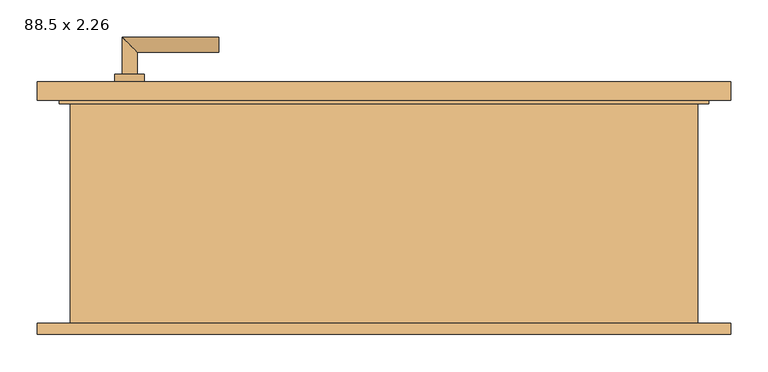
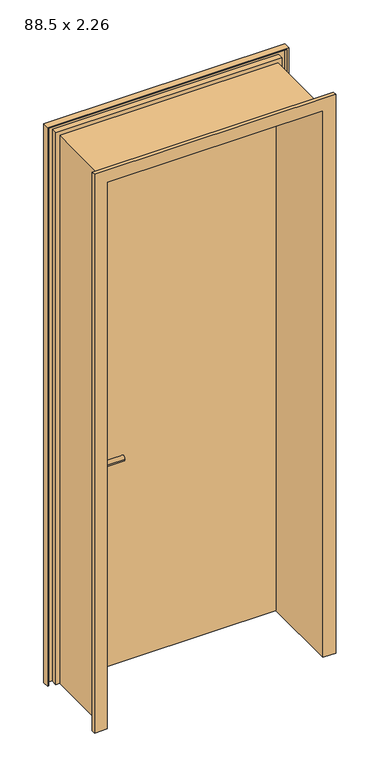
"""IFC4 building model written with IfcOpenShell, lengths in millimetres: door geometry, Drehflügel 1-flg - Stahlzarge : 88.5 x 2.26."""

from ifc_helpers import new_model, si_unit, point, frame, frame_2d, origin, place, context, project, spatial, polyline, circle_curve, ellipse_curve, trimmed, segment, composite_curve, outline, extrude, faceted_brep, source, transform, mapped, element, save
from ifc_brep_helpers import plane_surface, cylinder_surface, advanced_brep


def door_88_5_x_2_26_ba7bfb9e(model_context):
    return source(origin(), model_context, "Body", "SolidModel", [
        advanced_brep(
        [(-352.5, 139.4346141, 1000.0), (-332.5, 139.4346141, 1000.0), (-352.5, 69.4346141, 1000.0), (-332.5, 89.4346141, 1000.0), (-222.5, 69.4346141, 1000.0), (-222.5, 89.4346141, 1000.0)],
        [
            (0, 1, circle_curve(frame((-342.5, 139.4346141, 1000.0), z_axis=(0.0, 1.0, 0.0), x_axis=(1.0, 0.0, 0.0)), 10.0)),
            (1, 0, circle_curve(frame((-342.5, 139.4346141, 1000.0), z_axis=(0.0, 1.0, 0.0), x_axis=(1.0, 0.0, 0.0)), 10.0)),
            (0, 2),
            (2, 3, ellipse_curve(frame((-342.5, 79.4346141, 1000.0), z_axis=(-0.7071067811865385, 0.7071067811865565, 0.0), x_axis=(0.7071067811865563, 0.7071067811865386, 0.0)), 14.1421356, 10.0)),
            (3, 1),
            (3, 2, ellipse_curve(frame((-342.5, 79.4346141, 1000.0), z_axis=(-0.7071067811865385, 0.7071067811865565, 0.0), x_axis=(0.7071067811865563, 0.7071067811865386, 0.0)), 14.1421356, 10.0)),
            (4, 5, circle_curve(frame((-222.5, 79.4346141, 1000.0), z_axis=(1.0, 0.0, 0.0), x_axis=(0.0, 1.0, 0.0)), 10.0)),
            (5, 4, circle_curve(frame((-222.5, 79.4346141, 1000.0), z_axis=(1.0, 0.0, 0.0), x_axis=(0.0, 1.0, 0.0)), 10.0)),
            (2, 4),
            (5, 3),
        ],
        [
            plane_surface(frame((-342.5, 139.4346141, -287.7526403), z_axis=(0.0, 1.0, 0.0), x_axis=(0.0, 0.0, 1.0))),
            cylinder_surface(frame((-342.5, 139.4346141, 1000.0), z_axis=(0.0, 1.0, 0.0), x_axis=(1.0, 0.0, 0.0)), 10.0),
            plane_surface(frame((-222.5, 79.4346141, -287.7526403), z_axis=(1.0, 0.0, 0.0), x_axis=(0.0, 0.0, 1.0))),
            cylinder_surface(frame((-342.5, 79.4346141, 1000.0), z_axis=(-1.0, 0.0, 0.0), x_axis=(0.0, 1.0, 0.0)), 10.0),
        ],
        [
            (0, [[1, 2]]),
            (1, [[-1, 3, 4, 5]]),
            (1, [[-2, -5, 6, -3]]),
            (2, [[7, 8]]),
            (3, [[-4, 9, -8, 10]]),
            (3, [[-6, -10, -7, -9]]),
        ],
    ),
        advanced_brep(
        [(-332.5, 199.4346141, 1000.0), (-352.5, 199.4346141, 1000.0), (-332.5, 229.4346141, 1000.0), (-352.5, 249.4346141, 1000.0), (-222.5, 229.4346141, 1000.0), (-222.5, 249.4346141, 1000.0)],
        [
            (0, 1, circle_curve(frame((-342.5, 199.4346141, 1000.0), z_axis=(0.0, -1.0, 0.0), x_axis=(-1.0, 0.0, 0.0)), 10.0)),
            (1, 0, circle_curve(frame((-342.5, 199.4346141, 1000.0), z_axis=(0.0, -1.0, 0.0), x_axis=(-1.0, 0.0, 0.0)), 10.0)),
            (0, 2),
            (2, 3, ellipse_curve(frame((-342.5, 239.4346141, 1000.0), z_axis=(-0.7071067811865475, -0.7071067811865475, 0.0), x_axis=(0.7071067811865474, -0.7071067811865476, 0.0)), 14.1421356, 10.0)),
            (3, 1),
            (3, 2, ellipse_curve(frame((-342.5, 239.4346141, 1000.0), z_axis=(-0.7071067811865475, -0.7071067811865475, 0.0), x_axis=(0.7071067811865474, -0.7071067811865476, 0.0)), 14.1421356, 10.0)),
            (4, 5, circle_curve(frame((-222.5, 239.4346141, 1000.0), z_axis=(1.0, 0.0, 0.0), x_axis=(0.0, 1.0, 0.0)), 10.0)),
            (5, 4, circle_curve(frame((-222.5, 239.4346141, 1000.0), z_axis=(1.0, 0.0, 0.0), x_axis=(0.0, 1.0, 0.0)), 10.0)),
            (2, 4),
            (5, 3),
        ],
        [
            plane_surface(frame((-342.5, 199.4346141, -287.7526403), z_axis=(0.0, -1.0, 0.0), x_axis=(0.0, 0.0, 1.0))),
            cylinder_surface(frame((-342.5, 199.4346141, 1000.0), z_axis=(0.0, -1.0, 0.0), x_axis=(-1.0, 0.0, 0.0)), 10.0),
            plane_surface(frame((-222.5, 239.4346141, -287.7526403), z_axis=(1.0, 0.0, 0.0), x_axis=(0.0, 0.0, 1.0))),
            cylinder_surface(frame((-342.5, 239.4346141, 1000.0), z_axis=(-1.0, 0.0, 0.0), x_axis=(0.0, 1.0, 0.0)), 10.0),
        ],
        [
            (0, [[1, 2]]),
            (1, [[-1, 3, 4, 5]]),
            (1, [[-2, -5, 6, -3]]),
            (2, [[7, 8]]),
            (3, [[-4, 9, -8, 10]]),
            (3, [[-6, -10, -7, -9]]),
        ],
    ),
        extrude(outline(composite_curve([segment(trimmed(circle_curve(frame_2d((1000.0, -342.5)), 20.0), [point((1000.0, -362.5))], [point((1000.0, -322.5))], False, "CARTESIAN"), True, "CONTINUOUS"), segment(trimmed(circle_curve(frame_2d((1000.0, -342.5)), 20.0), [point((1000.0, -322.5))], [point((1000.0, -362.5))], False, "CARTESIAN"), True, "CONTINUOUS")], self_intersect=False)), frame((0.0, 129.4346141, 0.0), z_axis=(0.0, 1.0, 0.0), x_axis=(0.0, 0.0, 1.0)), (0.0, 0.0, 1.0), 10.0),
        extrude(outline(composite_curve([segment(trimmed(circle_curve(frame_2d((1000.0, -342.5)), 20.0), [point((1000.0, -362.5))], [point((1000.0, -322.5))], False, "CARTESIAN"), True, "CONTINUOUS"), segment(trimmed(circle_curve(frame_2d((1000.0, -342.5)), 20.0), [point((1000.0, -322.5))], [point((1000.0, -362.5))], False, "CARTESIAN"), True, "CONTINUOUS")], self_intersect=False)), frame((0.0, 189.4346141, 0.0), z_axis=(0.0, 1.0, 0.0), x_axis=(0.0, 0.0, 1.0)), (0.0, 0.0, 1.0), 10.0),
        extrude(outline(polyline([(432.5, 164.4346141), (-432.5, 164.4346141), (-432.5, 189.4346141), (432.5, 189.4346141), (432.5, 164.4346141)])), frame((0.0, 0.0, 100.0), z_axis=(0.0, 0.0, 1.0), x_axis=(1.0, 0.0, 0.0)), (0.0, 0.0, 1.0), 2250.0),
        faceted_brep([(466.9603207, -150.5653859, 100.0), (417.5, -150.5653859, 100.0), (417.5, 164.4346141, 100.0), (432.5, 164.4346141, 100.0), (432.5, 189.4346141, 100.0), (466.9603207, 189.4346141, 100.0), (466.9603207, 164.4346141, 100.0), (461.9603207, 164.4346141, 100.0), (461.9603207, 184.4346141, 100.0), (437.5, 184.4346141, 100.0), (437.5, 159.4346141, 100.0), (422.5, 159.4346141, 100.0), (422.5, -145.5653859, 100.0), (461.9603207, -145.5653859, 100.0), (461.9603207, -135.5653859, 100.0), (466.9603207, -135.5653859, 100.0), (466.9603207, -150.5653859, 2384.4603207), (-466.9603207, -150.5653859, 2384.4603207), (-466.9603207, -150.5653859, 100.0), (-417.5, -150.5653859, 100.0), (-417.5, -150.5653859, 2335.0), (417.5, -150.5653859, 2335.0), (417.5, 164.4346141, 2335.0), (-417.5, 164.4346141, 2335.0), (-417.5, 164.4346141, 100.0), (-432.5, 164.4346141, 100.0), (-432.5, 164.4346141, 2350.0), (432.5, 164.4346141, 2350.0), (432.5, 189.4346141, 2350.0), (-432.5, 189.4346141, 2350.0), (-432.5, 189.4346141, 100.0), (-466.9603207, 189.4346141, 100.0), (-466.9603207, 189.4346141, 2384.4603207), (466.9603207, 189.4346141, 2384.4603207), (466.9603207, 164.4346141, 2384.4603207), (-466.9603207, 164.4346141, 2384.4603207), (-466.9603207, 164.4346141, 100.0), (-461.9603207, 164.4346141, 100.0), (-461.9603207, 164.4346141, 2379.4603207), (461.9603207, 164.4346141, 2379.4603207), (461.9603207, 184.4346141, 2379.4603207), (-461.9603207, 184.4346141, 2379.4603207), (-461.9603207, 184.4346141, 100.0), (-437.5, 184.4346141, 100.0), (-437.5, 184.4346141, 2355.0), (437.5, 184.4346141, 2355.0), (437.5, 159.4346141, 2355.0), (-437.5, 159.4346141, 2355.0), (-437.5, 159.4346141, 100.0), (-422.5, 159.4346141, 100.0), (-422.5, 159.4346141, 2340.0), (422.5, 159.4346141, 2340.0), (422.5, -145.5653859, 2340.0), (-422.5, -145.5653859, 2340.0), (-422.5, -145.5653859, 100.0), (-461.9603207, -145.5653859, 100.0), (-461.9603207, -145.5653859, 2379.4603207), (461.9603207, -145.5653859, 2379.4603207), (461.9603207, -135.5653859, 2379.4603207), (-461.9603207, -135.5653859, 2379.4603207), (-461.9603207, -135.5653859, 100.0), (-466.9603207, -135.5653859, 100.0), (-466.9603207, -135.5653859, 2384.4603207), (466.9603207, -135.5653859, 2384.4603207)], [[[0, 1, 2, 3, 4, 5, 6, 7, 8, 9, 10, 11, 12, 13, 14, 15]], [[1, 0, 16, 17, 18, 19, 20, 21]], [[2, 1, 21, 22]], [[3, 2, 22, 23, 24, 25, 26, 27]], [[4, 3, 27, 28]], [[5, 4, 28, 29, 30, 31, 32, 33]], [[6, 5, 33, 34]], [[7, 6, 34, 35, 36, 37, 38, 39]], [[8, 7, 39, 40]], [[9, 8, 40, 41, 42, 43, 44, 45]], [[10, 9, 45, 46]], [[11, 10, 46, 47, 48, 49, 50, 51]], [[12, 11, 51, 52]], [[13, 12, 52, 53, 54, 55, 56, 57]], [[14, 13, 57, 58]], [[15, 14, 58, 59, 60, 61, 62, 63]], [[0, 15, 63, 16]], [[17, 62, 61, 18]], [[18, 61, 60, 55, 54, 49, 48, 43, 42, 37, 36, 31, 30, 25, 24, 19]], [[23, 20, 19, 24]], [[29, 26, 25, 30]], [[35, 32, 31, 36]], [[41, 38, 37, 42]], [[47, 44, 43, 48]], [[53, 50, 49, 54]], [[59, 56, 55, 60]], [[22, 21, 20, 23]], [[28, 27, 26, 29]], [[34, 33, 32, 35]], [[40, 39, 38, 41]], [[46, 45, 44, 47]], [[52, 51, 50, 53]], [[58, 57, 56, 59]], [[16, 63, 62, 17]]]),
    ])


if __name__ == "__main__":
    model = new_model("IFC4")
    model_context = context("Model", 3, world=origin())
    ifc_project = project(units=[si_unit("LENGTHUNIT", "METRE", prefix="MILLI")], contexts=[model_context])
    site = spatial("IfcSite", under=ifc_project)
    building = spatial("IfcBuilding", under=site)
    placement = place(None, origin())
    door_88_5_x_2_26_shape = door_88_5_x_2_26_ba7bfb9e(model_context)
    element("IfcDoor", 1, ObjectType="Drehflügel 1-flg - Stahlzarge : 88.5 x 2.26", at=placement, inside=building, context=model_context, shape_type="MappedRepresentation", body=[
        mapped(door_88_5_x_2_26_shape, transform((0.0, 0.0, 0.0), x_axis=(1.0, 0.0, 0.0), y_axis=(0.0, 1.0, 0.0), z_axis=(0.0, 0.0, 1.0))),
    ])
    save(model, "model.ifc")

# Revit data of these elements
# Type "Drehflügel 1-flg - Stahlzarge : 88.5 x 2.26"
#   Construction Type Id = "MDOOR"
#   Type Mark = "20"
#   Operation = "SingleSwingRight"
#   Keynote = "16.03"
#   Analytic Construction = "Metall"
#   Thermal Resistance (R) = 0.270117 (m²·K)/W
#   Heat Transfer Coefficient (U) = 3.7021 W/(m²·K)
#   Rough Width = 0.885 m
#   Rough Height [instance default] = 2.360 m
#   Höhe Türgriff [instance default] = 0.900 m
#   Height = 2.260 m
#   Fußbodenaufbau [instance default] = 0.100 m
#   Width = 0.885 m
#   Sichtbarkeit Sturzlinien [instance default] = yes
#   Türgriff auswählen [instance default] = element 221079
#   Türgriff [instance default] = none
#   Türflügel [instance default] = none
#   Rahmen/Pfosten [instance default] = Metall - Lackiert - Grau
#   Visual Light Transmittance = 0
#   Solar Heat Gain Coefficient = 0
#   Function = (empty or 0)
#   Wall Closure = (empty or 0)
# Element 1 (IfcDoor, "Drehflügel 1-flg - Stahlzarge : 88.5 x 2.26")
#   Materials on its faces: "Metall - Lackiert - Grau", "Metall - Chrom", "Holz - Birke"
# Materials
#   "Metall - Lackiert - Grau": class "Farbe 1", colour RGB 98 98 98, transparency 0, Cost = 0
#   "Metall - Chrom": class "Metall", colour RGB 247 247 247, transparency 0, Cost = 0
#   "Holz - Birke": class "Holz", colour RGB 213 164 103, transparency 0, Cost = 0
